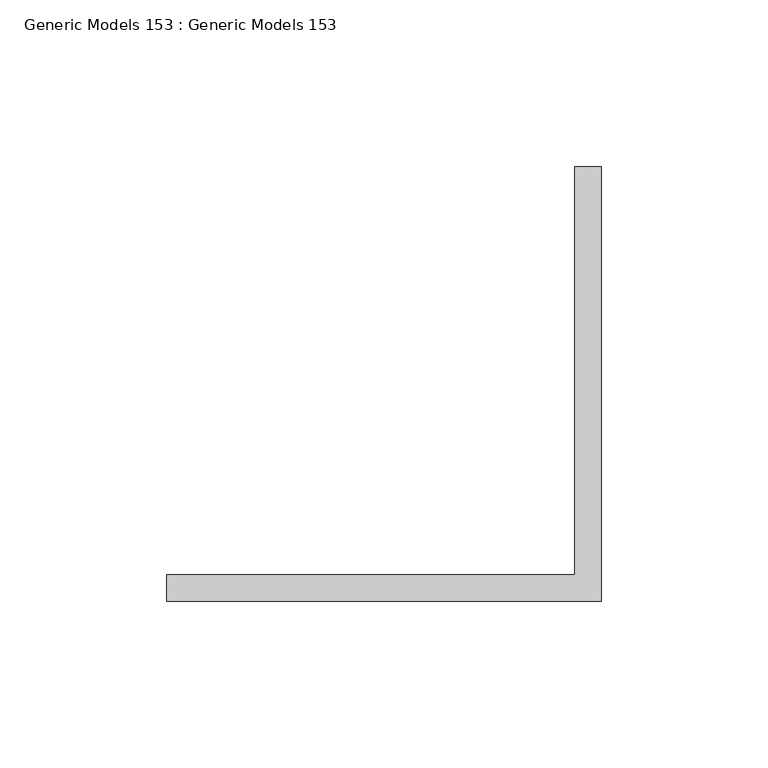
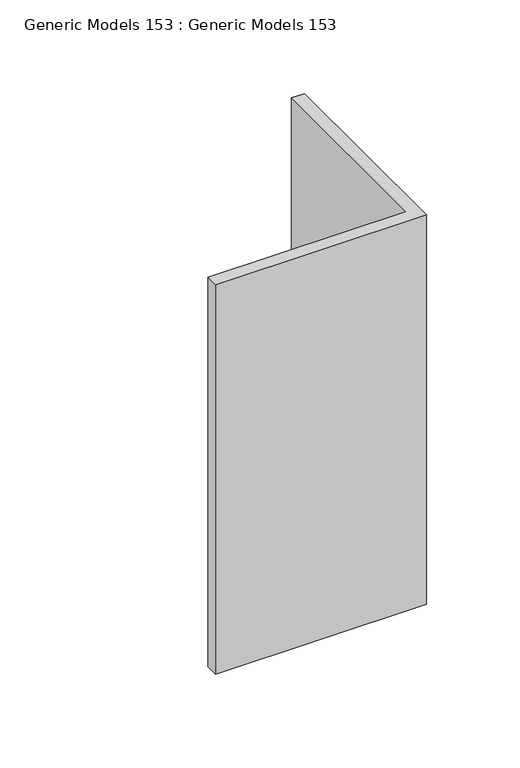
"""IFC4 building model written with IfcOpenShell, lengths in millimetres: proxy geometry, Generic Models 153 : Generic Models 153."""

from ifc_helpers import new_model, si_unit, frame, origin, place, context, project, spatial, polyline, outline, extrude, source, transform, mapped, element, save


def generic_models_153_generic_models_153_ea4ddf0c(model_context):
    return source(origin(), model_context, "Body", "SweptSolid", [
        extrude(outline(polyline([(31762.6846032, 36607.4457942), (31770.6221032, 36607.4457942), (31770.6221032, 36477.2707942), (31640.4471032, 36477.2707942), (31640.4471032, 36485.2082942), (31762.6846032, 36485.2082942), (31762.6846032, 36607.4457942)])), frame((0.0, 0.0, 271626.0125), z_axis=(0.0, 0.0, 1.0), x_axis=(1.0, 0.0, 0.0)), (0.0, 0.0, 1.0), 254.0),
    ])


if __name__ == "__main__":
    model = new_model("IFC4")
    model_context = context("Model", 3, world=origin())
    ifc_project = project(units=[si_unit("LENGTHUNIT", "METRE", prefix="MILLI")], contexts=[model_context])
    site = spatial("IfcSite", under=ifc_project)
    building = spatial("IfcBuilding", under=site)
    placement = place(None, origin())
    generic_models_153_generic_models_153_shape = generic_models_153_generic_models_153_ea4ddf0c(model_context)
    element("IfcBuildingElementProxy", 1, Name="Generic Models 153 : Generic Models 153", ObjectType="Generic Models 153 : Generic Models 153", at=placement, inside=building, context=model_context, shape_type="MappedRepresentation", body=[
        mapped(generic_models_153_generic_models_153_shape, transform((0.0, 0.0, 0.0), x_axis=(1.0, 0.0, 0.0), y_axis=(0.0, 1.0, 0.0), z_axis=(0.0, 0.0, 1.0))),
    ])
    save(model, "model.ifc")
